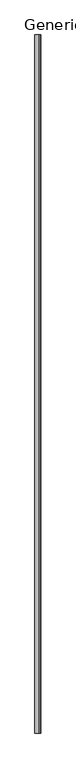
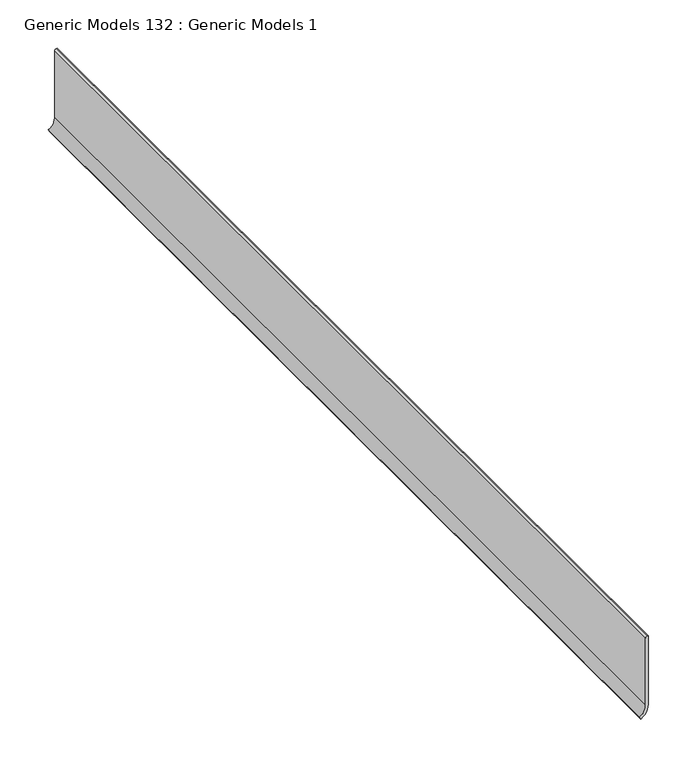
"""IFC4 building model written with IfcOpenShell, lengths in millimetres: proxy geometry, Generic Models 132 : Generic Models 1."""

from ifc_helpers import new_model, si_unit, point, frame, frame_2d, origin, place, context, project, spatial, polyline, circle_curve, trimmed, segment, composite_curve, outline, extrude, source, transform, mapped, element, save


def generic_models_132_generic_models_1_f536fb9f(model_context):
    return source(origin(), model_context, "Body", "SweptSolid", [
        extrude(outline(composite_curve([segment(polyline([(73.749588, 50688.3189813), (73.749588, 50687.2307831)]), True, "CONTINUOUS"), segment(trimmed(circle_curve(frame_2d((71.6627862, 50687.2307831)), 2.0868018), [point((73.749588, 50687.2307831))], [point((71.6627862, 50685.1439813))], False, "CARTESIAN"), True, "CONTINUOUS"), segment(polyline([(71.6627862, 50685.1439813), (-12.4007813, 50685.1439813)]), True, "CONTINUOUS"), segment(trimmed(circle_curve(frame_2d((-12.4007813, 50670.4792845)), 14.6646968), [point((-12.4007813, 50685.1439813))], [point((-25.1007813, 50677.8116329))], True, "CARTESIAN"), True, "CONTINUOUS"), segment(polyline([(-25.1007813, 50677.8116329), (-27.850412, 50679.3991329)]), True, "CONTINUOUS"), segment(trimmed(circle_curve(frame_2d((-12.4007813, 50670.4792845)), 17.8396968), [point((-27.850412, 50679.3991329))], [point((-12.4007813, 50688.3189813))], False, "CARTESIAN"), True, "CONTINUOUS"), segment(polyline([(-12.4007813, 50688.3189813), (73.749588, 50688.3189813)]), True, "CONTINUOUS")], self_intersect=False)), frame((0.0, 0.0, 0.0), z_axis=(0.0, 1.0, 0.0), x_axis=(0.0, 0.0, 1.0)), (0.0, 0.0, 1.0), 1219.2),
    ])


if __name__ == "__main__":
    model = new_model("IFC4")
    model_context = context("Model", 3, world=origin())
    ifc_project = project(units=[si_unit("LENGTHUNIT", "METRE", prefix="MILLI")], contexts=[model_context])
    site = spatial("IfcSite", under=ifc_project)
    building = spatial("IfcBuilding", under=site)
    placement = place(None, origin())
    generic_models_132_generic_models_1_shape = generic_models_132_generic_models_1_f536fb9f(model_context)
    element("IfcBuildingElementProxy", 1, Name="Generic Models 132 : Generic Models 1", ObjectType="Generic Models 132 : Generic Models 1", at=placement, inside=building, context=model_context, shape_type="MappedRepresentation", body=[
        mapped(generic_models_132_generic_models_1_shape, transform((0.0, 0.0, 0.0), x_axis=(1.0, 0.0, 0.0), y_axis=(0.0, 1.0, 0.0), z_axis=(0.0, 0.0, 1.0))),
    ])
    save(model, "model.ifc")

# Revit data of these elements
# Element 1 (IfcBuildingElementProxy, "Generic Models 132 : Generic Models 1")
#   Materials on its faces: "BASE AS SCHEDULED"
# Materials
#   "BASE AS SCHEDULED": class "Generic", colour RGB 120 120 120, transparency 0, Cost = 0
